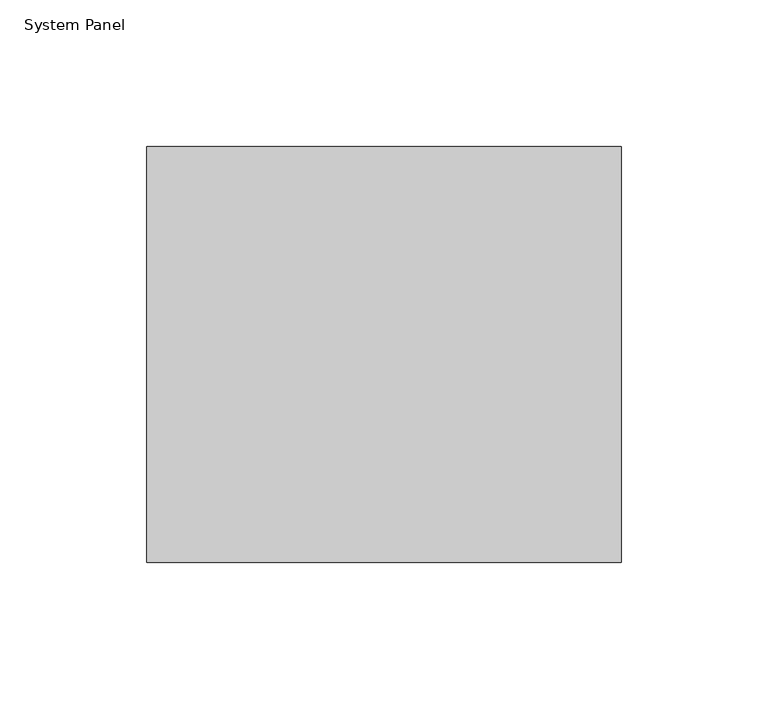
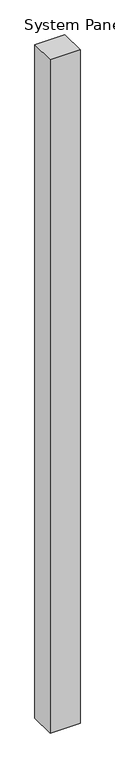
"""IFC4 building model written with IfcOpenShell, lengths in millimetres: plate geometry, System Panel : NLRS_21_CWP_hsb-vulling minerale wol 142 _gen_rsf."""

from ifc_helpers import new_model, si_unit, origin, origin_with_axes, place, context, project, spatial, polyline, outline, extrude, source, transform, mapped, element, save


def system_panel_9935ab3f(model_context):
    return source(origin(), model_context, "Body", "SweptSolid", [
        extrude(outline(polyline([(80.9999998, -71.0), (-80.9999998, -71.0), (-80.9999998, 71.0), (80.9999998, 71.0), (80.9999998, -71.0)])), origin_with_axes(), (0.0, 0.0, 1.0), 3849.0),
    ])


if __name__ == "__main__":
    model = new_model("IFC4")
    model_context = context("Model", 3, world=origin())
    ifc_project = project(units=[si_unit("LENGTHUNIT", "METRE", prefix="MILLI")], contexts=[model_context])
    site = spatial("IfcSite", under=ifc_project)
    building = spatial("IfcBuilding", under=site)
    placement = place(None, origin())
    system_panel_shape = system_panel_9935ab3f(model_context)
    element("IfcPlate", 1, ObjectType="System Panel : NLRS_21_CWP_hsb-vulling minerale wol 142 _gen_rsf", at=placement, inside=building, context=model_context, shape_type="MappedRepresentation", body=[
        mapped(system_panel_shape, transform((0.0, 0.0, 0.0), x_axis=(1.0, 0.0, 0.0), y_axis=(0.0, 1.0, 0.0), z_axis=(0.0, 0.0, 1.0))),
    ])
    save(model, "model.ifc")

# Revit data of these elements
# Type "System Panel : NLRS_21_CWP_hsb-vulling minerale wol 142 _gen_rsf"
#   Export Type to IFC As = "IfcWall"
#   Type IfcGUID = "07M7mRoiH1CR8m_RSKIwpC"
#   Assembly Code = "21.23"
# Element 1 (IfcPlate, "System Panel : NLRS_21_CWP_hsb-vulling minerale wol 142 _gen_rsf")
#   Materials on its faces: "NLRS_m1_isolatie minerale wol_gen_rsf"
# Materials
#   "NLRS_m1_isolatie minerale wol_gen_rsf": class "M - Anorganische materialen", colour RGB 200 200 140, transparency 0, Keynote = "m1", Manufacturer = "Revit Standards Foundation", URL = "www.revitstandards.org", Description = "isolatie minerale wol", Cost = 0
